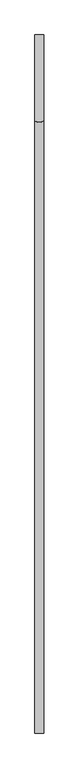
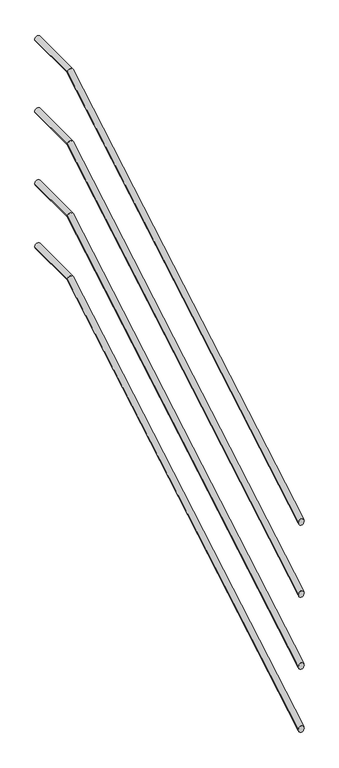
"""IFC4 building model written with IfcOpenShell, lengths in millimetres: railing geometry."""

from ifc_helpers import new_model, si_unit, frame, origin, place, context, project, spatial, circle_curve, ellipse_curve, source, transform, mapped, element, save
from ifc_brep_helpers import plane_surface, cylinder_surface, advanced_brep


def railing_f234ddb2(model_context):
    return source(origin(), model_context, "Body", "AdvancedBrep", [
        advanced_brep(
        [(-1890.4, 13399.5208589, 7257.5963084), (-1860.4, 13399.5208589, 7257.5963084), (-1890.4, 15503.576096, 8484.9618634), (-1860.4, 15503.576096, 8484.9618634), (-1890.4, 15799.5208589, 8484.9618634), (-1860.4, 15799.5208589, 8484.9618634)],
        [
            (0, 1, ellipse_curve(frame((-1875.4, 13399.5208589, 7257.5963084), z_axis=(0.0, -1.0, 0.0), x_axis=(0.0, 0.0, -1.0)), 17.365555, 15.0)),
            (1, 0, ellipse_curve(frame((-1875.4, 13399.5208589, 7257.5963084), z_axis=(0.0, -1.0, 0.0), x_axis=(0.0, 0.0, -1.0)), 17.365555, 15.0)),
            (0, 2),
            (2, 3, ellipse_curve(frame((-1875.4, 15503.576096, 8484.9618634), z_axis=(0.0, -0.965344213454049, -0.26097997921446653), x_axis=(0.0, 0.2609799792144656, -0.9653442134540494)), 15.5384989, 15.0)),
            (3, 1),
            (3, 2, ellipse_curve(frame((-1875.4, 15503.576096, 8484.9618634), z_axis=(0.0, -0.965344213454049, -0.26097997921446653), x_axis=(0.0, 0.2609799792144656, -0.9653442134540494)), 15.5384989, 15.0)),
            (4, 5, circle_curve(frame((-1875.4, 15799.5208589, 8484.9618634), z_axis=(0.0, 1.0, 0.0), x_axis=(1.0, 0.0, 0.0)), 15.0)),
            (5, 4, circle_curve(frame((-1875.4, 15799.5208589, 8484.9618634), z_axis=(0.0, 1.0, 0.0), x_axis=(1.0, 0.0, 0.0)), 15.0)),
            (2, 4),
            (5, 3),
        ],
        [
            plane_surface(frame((-1875.4, 13399.5208589, 7274.9618634), z_axis=(0.0, -1.0, 0.0), x_axis=(0.0, 0.0, 1.0))),
            cylinder_surface(frame((-1875.4, 13407.0789243, 7262.0051799), z_axis=(0.0, -0.8637789008984332, -0.5038710255240865), x_axis=(1.0, 0.0, 0.0)), 15.0),
            plane_surface(frame((-1875.4, 15799.5208589, 8499.9618634), z_axis=(0.0, 1.0, 0.0), x_axis=(0.0, 0.0, 1.0))),
            cylinder_surface(frame((-1875.4, 15499.5208589, 8484.9618634), z_axis=(0.0, -1.0, 0.0), x_axis=(1.0, 0.0, 0.0)), 15.0),
        ],
        [
            (0, [[1, 2]]),
            (1, [[-1, 3, 4, 5]]),
            (1, [[-2, -5, 6, -3]]),
            (2, [[7, 8]]),
            (3, [[-4, 9, -8, 10]]),
            (3, [[-6, -10, -7, -9]]),
        ],
    ),
        advanced_brep(
        [(-1890.4, 13399.5208589, 6457.5963084), (-1860.4, 13399.5208589, 6457.5963084), (-1890.4, 15503.576096, 7684.9618634), (-1860.4, 15503.576096, 7684.9618634), (-1890.4, 15799.5208589, 7684.9618634), (-1860.4, 15799.5208589, 7684.9618634)],
        [
            (0, 1, ellipse_curve(frame((-1875.4, 13399.5208589, 6457.5963084), z_axis=(0.0, -1.0, 0.0), x_axis=(0.0, 0.0, -1.0)), 17.365555, 15.0)),
            (1, 0, ellipse_curve(frame((-1875.4, 13399.5208589, 6457.5963084), z_axis=(0.0, -1.0, 0.0), x_axis=(0.0, 0.0, -1.0)), 17.365555, 15.0)),
            (0, 2),
            (2, 3, ellipse_curve(frame((-1875.4, 15503.576096, 7684.9618634), z_axis=(0.0, -0.965344213454049, -0.26097997921446653), x_axis=(0.0, 0.2609799792144656, -0.9653442134540494)), 15.5384989, 15.0)),
            (3, 1),
            (3, 2, ellipse_curve(frame((-1875.4, 15503.576096, 7684.9618634), z_axis=(0.0, -0.965344213454049, -0.26097997921446653), x_axis=(0.0, 0.2609799792144656, -0.9653442134540494)), 15.5384989, 15.0)),
            (4, 5, circle_curve(frame((-1875.4, 15799.5208589, 7684.9618634), z_axis=(0.0, 1.0, 0.0), x_axis=(1.0, 0.0, 0.0)), 15.0)),
            (5, 4, circle_curve(frame((-1875.4, 15799.5208589, 7684.9618634), z_axis=(0.0, 1.0, 0.0), x_axis=(1.0, 0.0, 0.0)), 15.0)),
            (2, 4),
            (5, 3),
        ],
        [
            plane_surface(frame((-1875.4, 13399.5208589, 6474.9618634), z_axis=(0.0, -1.0, 0.0), x_axis=(0.0, 0.0, 1.0))),
            cylinder_surface(frame((-1875.4, 13407.0789243, 6462.0051799), z_axis=(0.0, -0.8637789008984332, -0.5038710255240865), x_axis=(1.0, 0.0, 0.0)), 15.0),
            plane_surface(frame((-1875.4, 15799.5208589, 7699.9618634), z_axis=(0.0, 1.0, 0.0), x_axis=(0.0, 0.0, 1.0))),
            cylinder_surface(frame((-1875.4, 15499.5208589, 7684.9618634), z_axis=(0.0, -1.0, 0.0), x_axis=(1.0, 0.0, 0.0)), 15.0),
        ],
        [
            (0, [[1, 2]]),
            (1, [[-1, 3, 4, 5]]),
            (1, [[-2, -5, 6, -3]]),
            (2, [[7, 8]]),
            (3, [[-4, 9, -8, 10]]),
            (3, [[-6, -10, -7, -9]]),
        ],
    ),
        advanced_brep(
        [(-1890.4, 13399.5208589, 6857.5963084), (-1860.4, 13399.5208589, 6857.5963084), (-1890.4, 15503.576096, 8084.9618634), (-1860.4, 15503.576096, 8084.9618634), (-1890.4, 15799.5208589, 8084.9618634), (-1860.4, 15799.5208589, 8084.9618634)],
        [
            (0, 1, ellipse_curve(frame((-1875.4, 13399.5208589, 6857.5963084), z_axis=(0.0, -1.0, 0.0), x_axis=(0.0, 0.0, -1.0)), 17.365555, 15.0)),
            (1, 0, ellipse_curve(frame((-1875.4, 13399.5208589, 6857.5963084), z_axis=(0.0, -1.0, 0.0), x_axis=(0.0, 0.0, -1.0)), 17.365555, 15.0)),
            (0, 2),
            (2, 3, ellipse_curve(frame((-1875.4, 15503.576096, 8084.9618634), z_axis=(0.0, -0.965344213454049, -0.26097997921446653), x_axis=(0.0, 0.2609799792144656, -0.9653442134540494)), 15.5384989, 15.0)),
            (3, 1),
            (3, 2, ellipse_curve(frame((-1875.4, 15503.576096, 8084.9618634), z_axis=(0.0, -0.965344213454049, -0.26097997921446653), x_axis=(0.0, 0.2609799792144656, -0.9653442134540494)), 15.5384989, 15.0)),
            (4, 5, circle_curve(frame((-1875.4, 15799.5208589, 8084.9618634), z_axis=(0.0, 1.0, 0.0), x_axis=(1.0, 0.0, 0.0)), 15.0)),
            (5, 4, circle_curve(frame((-1875.4, 15799.5208589, 8084.9618634), z_axis=(0.0, 1.0, 0.0), x_axis=(1.0, 0.0, 0.0)), 15.0)),
            (2, 4),
            (5, 3),
        ],
        [
            plane_surface(frame((-1875.4, 13399.5208589, 6874.9618634), z_axis=(0.0, -1.0, 0.0), x_axis=(0.0, 0.0, 1.0))),
            cylinder_surface(frame((-1875.4, 13407.0789243, 6862.0051799), z_axis=(0.0, -0.8637789008984332, -0.5038710255240865), x_axis=(1.0, 0.0, 0.0)), 15.0),
            plane_surface(frame((-1875.4, 15799.5208589, 8099.9618634), z_axis=(0.0, 1.0, 0.0), x_axis=(0.0, 0.0, 1.0))),
            cylinder_surface(frame((-1875.4, 15499.5208589, 8084.9618634), z_axis=(0.0, -1.0, 0.0), x_axis=(1.0, 0.0, 0.0)), 15.0),
        ],
        [
            (0, [[1, 2]]),
            (1, [[-1, 3, 4, 5]]),
            (1, [[-2, -5, 6, -3]]),
            (2, [[7, 8]]),
            (3, [[-4, 9, -8, 10]]),
            (3, [[-6, -10, -7, -9]]),
        ],
    ),
        advanced_brep(
        [(-1890.4, 13399.5208589, 6107.5963084), (-1860.4, 13399.5208589, 6107.5963084), (-1890.4, 15503.576096, 7334.9618634), (-1860.4, 15503.576096, 7334.9618634), (-1890.4, 15799.5208589, 7334.9618634), (-1860.4, 15799.5208589, 7334.9618634)],
        [
            (0, 1, ellipse_curve(frame((-1875.4, 13399.5208589, 6107.5963084), z_axis=(0.0, -1.0, 0.0), x_axis=(0.0, 0.0, -1.0)), 17.365555, 15.0)),
            (1, 0, ellipse_curve(frame((-1875.4, 13399.5208589, 6107.5963084), z_axis=(0.0, -1.0, 0.0), x_axis=(0.0, 0.0, -1.0)), 17.365555, 15.0)),
            (0, 2),
            (2, 3, ellipse_curve(frame((-1875.4, 15503.576096, 7334.9618634), z_axis=(0.0, -0.965344213454049, -0.26097997921446653), x_axis=(0.0, 0.2609799792144656, -0.9653442134540494)), 15.5384989, 15.0)),
            (3, 1),
            (3, 2, ellipse_curve(frame((-1875.4, 15503.576096, 7334.9618634), z_axis=(0.0, -0.965344213454049, -0.26097997921446653), x_axis=(0.0, 0.2609799792144656, -0.9653442134540494)), 15.5384989, 15.0)),
            (4, 5, circle_curve(frame((-1875.4, 15799.5208589, 7334.9618634), z_axis=(0.0, 1.0, 0.0), x_axis=(1.0, 0.0, 0.0)), 15.0)),
            (5, 4, circle_curve(frame((-1875.4, 15799.5208589, 7334.9618634), z_axis=(0.0, 1.0, 0.0), x_axis=(1.0, 0.0, 0.0)), 15.0)),
            (2, 4),
            (5, 3),
        ],
        [
            plane_surface(frame((-1875.4, 13399.5208589, 6124.9618634), z_axis=(0.0, -1.0, 0.0), x_axis=(0.0, 0.0, 1.0))),
            cylinder_surface(frame((-1875.4, 13407.0789243, 6112.0051799), z_axis=(0.0, -0.8637789008984332, -0.5038710255240865), x_axis=(1.0, 0.0, 0.0)), 15.0),
            plane_surface(frame((-1875.4, 15799.5208589, 7349.9618634), z_axis=(0.0, 1.0, 0.0), x_axis=(0.0, 0.0, 1.0))),
            cylinder_surface(frame((-1875.4, 15499.5208589, 7334.9618634), z_axis=(0.0, -1.0, 0.0), x_axis=(1.0, 0.0, 0.0)), 15.0),
        ],
        [
            (0, [[1, 2]]),
            (1, [[-1, 3, 4, 5]]),
            (1, [[-2, -5, 6, -3]]),
            (2, [[7, 8]]),
            (3, [[-4, 9, -8, 10]]),
            (3, [[-6, -10, -7, -9]]),
        ],
    ),
    ])


if __name__ == "__main__":
    model = new_model("IFC4")
    model_context = context("Model", 3, world=origin())
    ifc_project = project(units=[si_unit("LENGTHUNIT", "METRE", prefix="MILLI")], contexts=[model_context])
    site = spatial("IfcSite", under=ifc_project)
    building = spatial("IfcBuilding", under=site)
    placement = place(None, origin())
    railing_shape = railing_f234ddb2(model_context)
    element("IfcRailing", 1, at=placement, inside=building, context=model_context, shape_type="MappedRepresentation", body=[
        mapped(railing_shape, transform((0.0, 0.0, 0.0), x_axis=(1.0, 0.0, 0.0), y_axis=(0.0, 1.0, 0.0), z_axis=(0.0, 0.0, 1.0))),
    ])
    save(model, "model.ifc")
